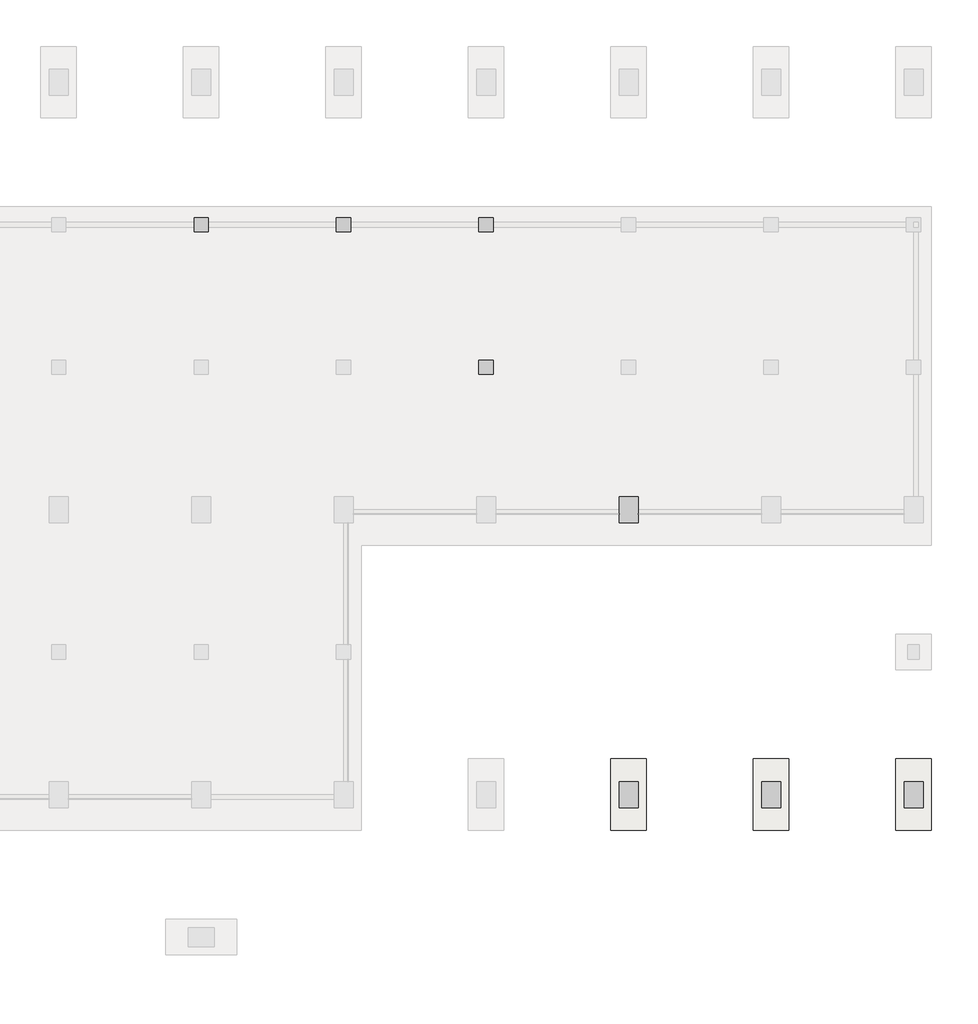
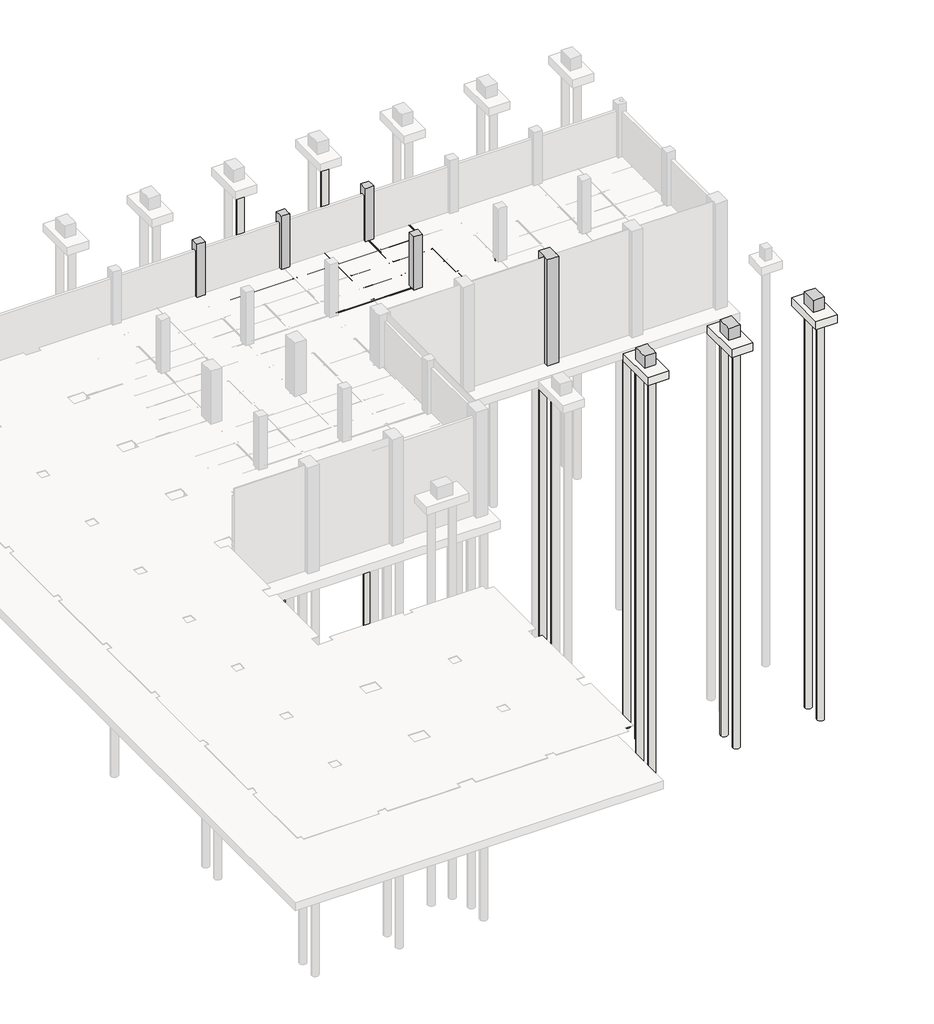
# Not in any storey, part 14 of 16: 21 beams, 17 slabs, 8 columns.
"""IFC4 building model written with IfcOpenShell, lengths in millimetres."""

from ifc_helpers import new_model, si_unit, point, frame, frame_2d, origin, place, context, project, spatial, polyline, circle_curve, trimmed, segment, composite_curve, outline, extrude, faceted_brep, element, save

model = new_model("IFC4")

# Units and contexts
model_context = context("Model", 3, world=origin())
ifc_project = project(units=[si_unit("LENGTHUNIT", "METRE", prefix="MILLI")], contexts=[model_context])

# Site, building
site = spatial("IfcSite", under=ifc_project)
building = spatial("IfcBuilding", under=site)

# Beams
placement = place(None, origin())
element("IfcBeam", 1, ObjectType="Steel Framing_C_KS : H_SB_AR_S02_C-150x75x6.5x10_J1", at=placement, inside=building, context=model_context, shape_type="SweptSolid", body=[
    extrude(outline(composite_curve([segment(polyline([(-7477.2, -3800.0381366), (-7477.2, -3950.0381366), (-7552.2, -3950.0381366)]), True, "CONTINUOUS"), segment(trimmed(circle_curve(frame_2d((-7542.2, -3950.0381366)), 10.0), [point((-7552.2, -3950.0381366))], [point((-7542.2, -3940.0381366))], False, "CARTESIAN"), True, "CONTINUOUS"), segment(polyline([(-7542.2, -3940.0381366), (-7483.7, -3930.7726469), (-7483.7, -3819.3036264), (-7542.2, -3810.0381366)]), True, "CONTINUOUS"), segment(trimmed(circle_curve(frame_2d((-7542.2, -3800.0381366)), 10.0), [point((-7542.2, -3810.0381366))], [point((-7552.2, -3800.0381366))], False, "CARTESIAN"), True, "CONTINUOUS"), segment(polyline([(-7552.2, -3800.0381366), (-7477.2, -3800.0381366)]), True, "CONTINUOUS")], self_intersect=False)), frame((48112.7, 0.0, 0.0), z_axis=(1.0, 0.0, 0.0), x_axis=(0.0, 1.0, 0.0)), (0.0, 0.0, 1.0), 2774.6),
])
element("IfcBeam", 2, ObjectType="Steel Framing_C_KS : H_SB_AR_S02_C-150x75x6.5x10_J1", at=placement, inside=building, context=model_context, shape_type="SweptSolid", body=[
    extrude(outline(composite_curve([segment(polyline([(-7477.2, -3800.0381366), (-7477.2, -3950.0381366), (-7552.2, -3950.0381366)]), True, "CONTINUOUS"), segment(trimmed(circle_curve(frame_2d((-7542.2, -3950.0381366)), 10.0), [point((-7552.2, -3950.0381366))], [point((-7542.2, -3940.0381366))], False, "CARTESIAN"), True, "CONTINUOUS"), segment(polyline([(-7542.2, -3940.0381366), (-7483.7, -3930.7726469), (-7483.7, -3819.3036264), (-7542.2, -3810.0381366)]), True, "CONTINUOUS"), segment(trimmed(circle_curve(frame_2d((-7542.2, -3800.0381366)), 10.0), [point((-7542.2, -3810.0381366))], [point((-7552.2, -3800.0381366))], False, "CARTESIAN"), True, "CONTINUOUS"), segment(polyline([(-7552.2, -3800.0381366), (-7477.2, -3800.0381366)]), True, "CONTINUOUS")], self_intersect=False)), frame((51112.7, 0.0, 0.0), z_axis=(1.0, 0.0, 0.0), x_axis=(0.0, 1.0, 0.0)), (0.0, 0.0, 1.0), 2774.6),
])
element("IfcBeam", 3, ObjectType="Steel Framing_H_KS : H_SB_AR_S02_H-400x200x8x13_BSG1", at=placement, inside=building, context=model_context, shape_type="SweptSolid", body=[
    extrude(outline(composite_curve([segment(polyline([(-11900.0, -4187.0381366), (-11900.0, -4200.0381366), (-12100.0, -4200.0381366), (-12100.0, -4187.0381366), (-12020.0, -4187.0381366)]), True, "CONTINUOUS"), segment(trimmed(circle_curve(frame_2d((-12020.0, -4171.0381366)), 16.0), [point((-12020.0, -4187.0381366))], [point((-12004.0, -4171.0381366))], True, "CARTESIAN"), True, "CONTINUOUS"), segment(polyline([(-12004.0, -4171.0381366), (-12004.0, -3829.0381366)]), True, "CONTINUOUS"), segment(trimmed(circle_curve(frame_2d((-12020.0, -3829.0381366)), 16.0), [point((-12004.0, -3829.0381366))], [point((-12020.0, -3813.0381366))], True, "CARTESIAN"), True, "CONTINUOUS"), segment(polyline([(-12020.0, -3813.0381366), (-12100.0, -3813.0381366), (-12100.0, -3800.0381366), (-11900.0, -3800.0381366), (-11900.0, -3813.0381366), (-11980.0, -3813.0381366)]), True, "CONTINUOUS"), segment(trimmed(circle_curve(frame_2d((-11980.0, -3829.0381366)), 16.0), [point((-11980.0, -3813.0381366))], [point((-11996.0, -3829.0381366))], True, "CARTESIAN"), True, "CONTINUOUS"), segment(polyline([(-11996.0, -3829.0381366), (-11996.0, -4171.0381366)]), True, "CONTINUOUS"), segment(trimmed(circle_curve(frame_2d((-11980.0, -4171.0381366)), 16.0), [point((-11996.0, -4171.0381366))], [point((-11980.0, -4187.0381366))], True, "CARTESIAN"), True, "CONTINUOUS"), segment(polyline([(-11980.0, -4187.0381366), (-11900.0, -4187.0381366)]), True, "CONTINUOUS")], self_intersect=False)), frame((54312.7, 0.0, 0.0), z_axis=(1.0, 0.0, 0.0), x_axis=(0.0, 1.0, 0.0)), (0.0, 0.0, 1.0), 5374.6),
])
element("IfcBeam", 4, ObjectType="Steel Framing_H_KS : H_SB_AR_S02_H-400x200x8x13_BSG2", at=placement, inside=building, context=model_context, shape_type="SweptSolid", body=[
    extrude(outline(composite_curve([segment(polyline([(-4187.0381366, 59900.0), (-4200.0381366, 59900.0), (-4200.0381366, 60100.0), (-4187.0381366, 60100.0), (-4187.0381366, 60020.0)]), True, "CONTINUOUS"), segment(trimmed(circle_curve(frame_2d((-4171.0381366, 60020.0)), 16.0), [point((-4187.0381366, 60020.0))], [point((-4171.0381366, 60004.0))], True, "CARTESIAN"), True, "CONTINUOUS"), segment(polyline([(-4171.0381366, 60004.0), (-3829.0381366, 60004.0)]), True, "CONTINUOUS"), segment(trimmed(circle_curve(frame_2d((-3829.0381366, 60020.0)), 16.0), [point((-3829.0381366, 60004.0))], [point((-3813.0381366, 60020.0))], True, "CARTESIAN"), True, "CONTINUOUS"), segment(polyline([(-3813.0381366, 60020.0), (-3813.0381366, 60100.0), (-3800.0381366, 60100.0), (-3800.0381366, 59900.0), (-3813.0381366, 59900.0), (-3813.0381366, 59980.0)]), True, "CONTINUOUS"), segment(trimmed(circle_curve(frame_2d((-3829.0381366, 59980.0)), 16.0), [point((-3813.0381366, 59980.0))], [point((-3829.0381366, 59996.0))], True, "CARTESIAN"), True, "CONTINUOUS"), segment(polyline([(-3829.0381366, 59996.0), (-4171.0381366, 59996.0)]), True, "CONTINUOUS"), segment(trimmed(circle_curve(frame_2d((-4171.0381366, 59980.0)), 16.0), [point((-4171.0381366, 59996.0))], [point((-4187.0381366, 59980.0))], True, "CARTESIAN"), True, "CONTINUOUS"), segment(polyline([(-4187.0381366, 59980.0), (-4187.0381366, 59900.0)]), True, "CONTINUOUS")], self_intersect=False)), frame((0.0, -11687.3, 0.0), z_axis=(0.0, 1.0, 0.0), x_axis=(0.0, 0.0, 1.0)), (0.0, 0.0, 1.0), 5374.6),
])
element("IfcBeam", 5, ObjectType="Steel Framing_H_KS : H_SB_AR_S02_H-400x200x8x13_BSB1", at=placement, inside=building, context=model_context, shape_type="SweptSolid", body=[
    extrude(outline(composite_curve([segment(polyline([(-4187.0381366, 56900.0), (-4200.0381366, 56900.0), (-4200.0381366, 57100.0), (-4187.0381366, 57100.0), (-4187.0381366, 57020.0)]), True, "CONTINUOUS"), segment(trimmed(circle_curve(frame_2d((-4171.0381366, 57020.0)), 16.0), [point((-4187.0381366, 57020.0))], [point((-4171.0381366, 57004.0))], True, "CARTESIAN"), True, "CONTINUOUS"), segment(polyline([(-4171.0381366, 57004.0), (-3829.0381366, 57004.0)]), True, "CONTINUOUS"), segment(trimmed(circle_curve(frame_2d((-3829.0381366, 57020.0)), 16.0), [point((-3829.0381366, 57004.0))], [point((-3813.0381366, 57020.0))], True, "CARTESIAN"), True, "CONTINUOUS"), segment(polyline([(-3813.0381366, 57020.0), (-3813.0381366, 57100.0), (-3800.0381366, 57100.0), (-3800.0381366, 56900.0), (-3813.0381366, 56900.0), (-3813.0381366, 56980.0)]), True, "CONTINUOUS"), segment(trimmed(circle_curve(frame_2d((-3829.0381366, 56980.0)), 16.0), [point((-3813.0381366, 56980.0))], [point((-3829.0381366, 56996.0))], True, "CARTESIAN"), True, "CONTINUOUS"), segment(polyline([(-3829.0381366, 56996.0), (-4171.0381366, 56996.0)]), True, "CONTINUOUS"), segment(trimmed(circle_curve(frame_2d((-4171.0381366, 56980.0)), 16.0), [point((-4171.0381366, 56996.0))], [point((-4187.0381366, 56980.0))], True, "CARTESIAN"), True, "CONTINUOUS"), segment(polyline([(-4187.0381366, 56980.0), (-4187.0381366, 56900.0)]), True, "CONTINUOUS")], self_intersect=False)), frame((0.0, -11887.3, 0.0), z_axis=(0.0, 1.0, 0.0), x_axis=(0.0, 0.0, 1.0)), (0.0, 0.0, 1.0), 5887.3),
])
element("IfcBeam", 6, ObjectType="Steel Framing_C_KS : H_SB_AR_S02_C-150x75x6.5x10_J1", at=placement, inside=building, context=model_context, shape_type="SweptSolid", body=[
    extrude(outline(composite_curve([segment(polyline([(-7477.2, -3800.0381366), (-7477.2, -3950.0381366), (-7552.2, -3950.0381366)]), True, "CONTINUOUS"), segment(trimmed(circle_curve(frame_2d((-7542.2, -3950.0381366)), 10.0), [point((-7552.2, -3950.0381366))], [point((-7542.2, -3940.0381366))], False, "CARTESIAN"), True, "CONTINUOUS"), segment(polyline([(-7542.2, -3940.0381366), (-7483.7, -3930.7726469), (-7483.7, -3819.3036264), (-7542.2, -3810.0381366)]), True, "CONTINUOUS"), segment(trimmed(circle_curve(frame_2d((-7542.2, -3800.0381366)), 10.0), [point((-7542.2, -3810.0381366))], [point((-7552.2, -3800.0381366))], False, "CARTESIAN"), True, "CONTINUOUS"), segment(polyline([(-7552.2, -3800.0381366), (-7477.2, -3800.0381366)]), True, "CONTINUOUS")], self_intersect=False)), frame((54112.7, 0.0, 0.0), z_axis=(1.0, 0.0, 0.0), x_axis=(0.0, 1.0, 0.0)), (0.0, 0.0, 1.0), 2774.6),
])
element("IfcBeam", 7, ObjectType="Steel Framing_C_KS : H_SB_AR_S02_C-150x75x6.5x10_J1", at=placement, inside=building, context=model_context, shape_type="SweptSolid", body=[
    extrude(outline(composite_curve([segment(polyline([(-8977.2, -3800.0381366), (-8977.2, -3950.0381366), (-9052.2, -3950.0381366)]), True, "CONTINUOUS"), segment(trimmed(circle_curve(frame_2d((-9042.2, -3950.0381366)), 10.0), [point((-9052.2, -3950.0381366))], [point((-9042.2, -3940.0381366))], False, "CARTESIAN"), True, "CONTINUOUS"), segment(polyline([(-9042.2, -3940.0381366), (-8983.7, -3930.7726469), (-8983.7, -3819.3036264), (-9042.2, -3810.0381366)]), True, "CONTINUOUS"), segment(trimmed(circle_curve(frame_2d((-9042.2, -3800.0381366)), 10.0), [point((-9042.2, -3810.0381366))], [point((-9052.2, -3800.0381366))], False, "CARTESIAN"), True, "CONTINUOUS"), segment(polyline([(-9052.2, -3800.0381366), (-8977.2, -3800.0381366)]), True, "CONTINUOUS")], self_intersect=False)), frame((57112.7, 0.0, 0.0), z_axis=(1.0, 0.0, 0.0), x_axis=(0.0, 1.0, 0.0)), (0.0, 0.0, 1.0), 2774.6),
])
element("IfcBeam", 8, ObjectType="Steel Framing_C_KS : H_SB_AR_S02_C-150x75x6.5x10_J1", at=placement, inside=building, context=model_context, shape_type="SweptSolid", body=[
    extrude(outline(composite_curve([segment(polyline([(-10477.2, -3800.0381366), (-10477.2, -3950.0381366), (-10552.2, -3950.0381366)]), True, "CONTINUOUS"), segment(trimmed(circle_curve(frame_2d((-10542.2, -3950.0381366)), 10.0), [point((-10552.2, -3950.0381366))], [point((-10542.2, -3940.0381366))], False, "CARTESIAN"), True, "CONTINUOUS"), segment(polyline([(-10542.2, -3940.0381366), (-10483.7, -3930.7726469), (-10483.7, -3819.3036264), (-10542.2, -3810.0381366)]), True, "CONTINUOUS"), segment(trimmed(circle_curve(frame_2d((-10542.2, -3800.0381366)), 10.0), [point((-10542.2, -3810.0381366))], [point((-10552.2, -3800.0381366))], False, "CARTESIAN"), True, "CONTINUOUS"), segment(polyline([(-10552.2, -3800.0381366), (-10477.2, -3800.0381366)]), True, "CONTINUOUS")], self_intersect=False)), frame((57112.7, 0.0, 0.0), z_axis=(1.0, 0.0, 0.0), x_axis=(0.0, 1.0, 0.0)), (0.0, 0.0, 1.0), 2774.6),
])
element("IfcBeam", 9, ObjectType="Steel Framing_C_KS : H_SB_AR_S02_C-150x75x6.5x10_J1", at=placement, inside=building, context=model_context, shape_type="SweptSolid", body=[
    extrude(outline(composite_curve([segment(polyline([(-7477.2, -3800.0381366), (-7477.2, -3950.0381366), (-7552.2, -3950.0381366)]), True, "CONTINUOUS"), segment(trimmed(circle_curve(frame_2d((-7542.2, -3950.0381366)), 10.0), [point((-7552.2, -3950.0381366))], [point((-7542.2, -3940.0381366))], False, "CARTESIAN"), True, "CONTINUOUS"), segment(polyline([(-7542.2, -3940.0381366), (-7483.7, -3930.7726469), (-7483.7, -3819.3036264), (-7542.2, -3810.0381366)]), True, "CONTINUOUS"), segment(trimmed(circle_curve(frame_2d((-7542.2, -3800.0381366)), 10.0), [point((-7542.2, -3810.0381366))], [point((-7552.2, -3800.0381366))], False, "CARTESIAN"), True, "CONTINUOUS"), segment(polyline([(-7552.2, -3800.0381366), (-7477.2, -3800.0381366)]), True, "CONTINUOUS")], self_intersect=False)), frame((57112.7, 0.0, 0.0), z_axis=(1.0, 0.0, 0.0), x_axis=(0.0, 1.0, 0.0)), (0.0, 0.0, 1.0), 2774.6),
])
element("IfcBeam", 10, ObjectType="Steel Framing_H_KS : H_SB_AR_S02_H-400x200x8x13_BSG1", at=placement, inside=building, context=model_context, shape_type="SweptSolid", body=[
    extrude(outline(composite_curve([segment(polyline([(-11900.0, -4187.0381366), (-11900.0, -4200.0381366), (-12100.0, -4200.0381366), (-12100.0, -4187.0381366), (-12020.0, -4187.0381366)]), True, "CONTINUOUS"), segment(trimmed(circle_curve(frame_2d((-12020.0, -4171.0381366)), 16.0), [point((-12020.0, -4187.0381366))], [point((-12004.0, -4171.0381366))], True, "CARTESIAN"), True, "CONTINUOUS"), segment(polyline([(-12004.0, -4171.0381366), (-12004.0, -3829.0381366)]), True, "CONTINUOUS"), segment(trimmed(circle_curve(frame_2d((-12020.0, -3829.0381366)), 16.0), [point((-12004.0, -3829.0381366))], [point((-12020.0, -3813.0381366))], True, "CARTESIAN"), True, "CONTINUOUS"), segment(polyline([(-12020.0, -3813.0381366), (-12100.0, -3813.0381366), (-12100.0, -3800.0381366), (-11900.0, -3800.0381366), (-11900.0, -3813.0381366), (-11980.0, -3813.0381366)]), True, "CONTINUOUS"), segment(trimmed(circle_curve(frame_2d((-11980.0, -3829.0381366)), 16.0), [point((-11980.0, -3813.0381366))], [point((-11996.0, -3829.0381366))], True, "CARTESIAN"), True, "CONTINUOUS"), segment(polyline([(-11996.0, -3829.0381366), (-11996.0, -4171.0381366)]), True, "CONTINUOUS"), segment(trimmed(circle_curve(frame_2d((-11980.0, -4171.0381366)), 16.0), [point((-11996.0, -4171.0381366))], [point((-11980.0, -4187.0381366))], True, "CARTESIAN"), True, "CONTINUOUS"), segment(polyline([(-11980.0, -4187.0381366), (-11900.0, -4187.0381366)]), True, "CONTINUOUS")], self_intersect=False)), frame((60312.7, 0.0, 0.0), z_axis=(1.0, 0.0, 0.0), x_axis=(0.0, 1.0, 0.0)), (0.0, 0.0, 1.0), 5374.6),
])
element("IfcBeam", 11, ObjectType="Steel Framing_H_KS : H_SB_AR_S02_H-400x200x8x13_BSB1", at=placement, inside=building, context=model_context, shape_type="SweptSolid", body=[
    extrude(outline(composite_curve([segment(polyline([(-4187.0381366, 62900.0), (-4200.0381366, 62900.0), (-4200.0381366, 63100.0), (-4187.0381366, 63100.0), (-4187.0381366, 63020.0)]), True, "CONTINUOUS"), segment(trimmed(circle_curve(frame_2d((-4171.0381366, 63020.0)), 16.0), [point((-4187.0381366, 63020.0))], [point((-4171.0381366, 63004.0))], True, "CARTESIAN"), True, "CONTINUOUS"), segment(polyline([(-4171.0381366, 63004.0), (-3829.0381366, 63004.0)]), True, "CONTINUOUS"), segment(trimmed(circle_curve(frame_2d((-3829.0381366, 63020.0)), 16.0), [point((-3829.0381366, 63004.0))], [point((-3813.0381366, 63020.0))], True, "CARTESIAN"), True, "CONTINUOUS"), segment(polyline([(-3813.0381366, 63020.0), (-3813.0381366, 63100.0), (-3800.0381366, 63100.0), (-3800.0381366, 62900.0), (-3813.0381366, 62900.0), (-3813.0381366, 62980.0)]), True, "CONTINUOUS"), segment(trimmed(circle_curve(frame_2d((-3829.0381366, 62980.0)), 16.0), [point((-3813.0381366, 62980.0))], [point((-3829.0381366, 62996.0))], True, "CARTESIAN"), True, "CONTINUOUS"), segment(polyline([(-3829.0381366, 62996.0), (-4171.0381366, 62996.0)]), True, "CONTINUOUS"), segment(trimmed(circle_curve(frame_2d((-4171.0381366, 62980.0)), 16.0), [point((-4171.0381366, 62996.0))], [point((-4187.0381366, 62980.0))], True, "CARTESIAN"), True, "CONTINUOUS"), segment(polyline([(-4187.0381366, 62980.0), (-4187.0381366, 62900.0)]), True, "CONTINUOUS")], self_intersect=False)), frame((0.0, -11887.3, 0.0), z_axis=(0.0, 1.0, 0.0), x_axis=(0.0, 0.0, 1.0)), (0.0, 0.0, 1.0), 5887.3),
])
element("IfcBeam", 12, ObjectType="Steel Framing_C_KS : H_SB_AR_S02_C-150x75x6.5x10_J1", at=placement, inside=building, context=model_context, shape_type="SweptSolid", body=[
    extrude(outline(composite_curve([segment(polyline([(-8977.2, -3800.0381366), (-8977.2, -3950.0381366), (-9052.2, -3950.0381366)]), True, "CONTINUOUS"), segment(trimmed(circle_curve(frame_2d((-9042.2, -3950.0381366)), 10.0), [point((-9052.2, -3950.0381366))], [point((-9042.2, -3940.0381366))], False, "CARTESIAN"), True, "CONTINUOUS"), segment(polyline([(-9042.2, -3940.0381366), (-8983.7, -3930.7726469), (-8983.7, -3819.3036264), (-9042.2, -3810.0381366)]), True, "CONTINUOUS"), segment(trimmed(circle_curve(frame_2d((-9042.2, -3800.0381366)), 10.0), [point((-9042.2, -3810.0381366))], [point((-9052.2, -3800.0381366))], False, "CARTESIAN"), True, "CONTINUOUS"), segment(polyline([(-9052.2, -3800.0381366), (-8977.2, -3800.0381366)]), True, "CONTINUOUS")], self_intersect=False)), frame((60112.7, 0.0, 0.0), z_axis=(1.0, 0.0, 0.0), x_axis=(0.0, 1.0, 0.0)), (0.0, 0.0, 1.0), 2774.6),
])
element("IfcBeam", 13, ObjectType="Steel Framing_C_KS : H_SB_AR_S02_C-150x75x6.5x10_J1", at=placement, inside=building, context=model_context, shape_type="SweptSolid", body=[
    extrude(outline(composite_curve([segment(polyline([(-10477.2, -3800.0381366), (-10477.2, -3950.0381366), (-10552.2, -3950.0381366)]), True, "CONTINUOUS"), segment(trimmed(circle_curve(frame_2d((-10542.2, -3950.0381366)), 10.0), [point((-10552.2, -3950.0381366))], [point((-10542.2, -3940.0381366))], False, "CARTESIAN"), True, "CONTINUOUS"), segment(polyline([(-10542.2, -3940.0381366), (-10483.7, -3930.7726469), (-10483.7, -3819.3036264), (-10542.2, -3810.0381366)]), True, "CONTINUOUS"), segment(trimmed(circle_curve(frame_2d((-10542.2, -3800.0381366)), 10.0), [point((-10542.2, -3810.0381366))], [point((-10552.2, -3800.0381366))], False, "CARTESIAN"), True, "CONTINUOUS"), segment(polyline([(-10552.2, -3800.0381366), (-10477.2, -3800.0381366)]), True, "CONTINUOUS")], self_intersect=False)), frame((60112.7, 0.0, 0.0), z_axis=(1.0, 0.0, 0.0), x_axis=(0.0, 1.0, 0.0)), (0.0, 0.0, 1.0), 2774.6),
])
element("IfcBeam", 14, ObjectType="Steel Framing_C_KS : H_SB_AR_S02_C-150x75x6.5x10_J1", at=placement, inside=building, context=model_context, shape_type="SweptSolid", body=[
    extrude(outline(composite_curve([segment(polyline([(-7477.2, -3800.0381366), (-7477.2, -3950.0381366), (-7552.2, -3950.0381366)]), True, "CONTINUOUS"), segment(trimmed(circle_curve(frame_2d((-7542.2, -3950.0381366)), 10.0), [point((-7552.2, -3950.0381366))], [point((-7542.2, -3940.0381366))], False, "CARTESIAN"), True, "CONTINUOUS"), segment(polyline([(-7542.2, -3940.0381366), (-7483.7, -3930.7726469), (-7483.7, -3819.3036264), (-7542.2, -3810.0381366)]), True, "CONTINUOUS"), segment(trimmed(circle_curve(frame_2d((-7542.2, -3800.0381366)), 10.0), [point((-7542.2, -3810.0381366))], [point((-7552.2, -3800.0381366))], False, "CARTESIAN"), True, "CONTINUOUS"), segment(polyline([(-7552.2, -3800.0381366), (-7477.2, -3800.0381366)]), True, "CONTINUOUS")], self_intersect=False)), frame((60112.7, 0.0, 0.0), z_axis=(1.0, 0.0, 0.0), x_axis=(0.0, 1.0, 0.0)), (0.0, 0.0, 1.0), 2774.6),
])
element("IfcBeam", 15, ObjectType="Steel Framing_H_KS : H_SB_AR_S02_H-400x200x8x13_BSG2", at=placement, inside=building, context=model_context, shape_type="SweptSolid", body=[
    extrude(outline(composite_curve([segment(polyline([(-4187.0381366, 59900.0), (-4200.0381366, 59900.0), (-4200.0381366, 60100.0), (-4187.0381366, 60100.0), (-4187.0381366, 60020.0)]), True, "CONTINUOUS"), segment(trimmed(circle_curve(frame_2d((-4171.0381366, 60020.0)), 16.0), [point((-4187.0381366, 60020.0))], [point((-4171.0381366, 60004.0))], True, "CARTESIAN"), True, "CONTINUOUS"), segment(polyline([(-4171.0381366, 60004.0), (-3829.0381366, 60004.0)]), True, "CONTINUOUS"), segment(trimmed(circle_curve(frame_2d((-3829.0381366, 60020.0)), 16.0), [point((-3829.0381366, 60004.0))], [point((-3813.0381366, 60020.0))], True, "CARTESIAN"), True, "CONTINUOUS"), segment(polyline([(-3813.0381366, 60020.0), (-3813.0381366, 60100.0), (-3800.0381366, 60100.0), (-3800.0381366, 59900.0), (-3813.0381366, 59900.0), (-3813.0381366, 59980.0)]), True, "CONTINUOUS"), segment(trimmed(circle_curve(frame_2d((-3829.0381366, 59980.0)), 16.0), [point((-3813.0381366, 59980.0))], [point((-3829.0381366, 59996.0))], True, "CARTESIAN"), True, "CONTINUOUS"), segment(polyline([(-3829.0381366, 59996.0), (-4171.0381366, 59996.0)]), True, "CONTINUOUS"), segment(trimmed(circle_curve(frame_2d((-4171.0381366, 59980.0)), 16.0), [point((-4171.0381366, 59996.0))], [point((-4187.0381366, 59980.0))], True, "CARTESIAN"), True, "CONTINUOUS"), segment(polyline([(-4187.0381366, 59980.0), (-4187.0381366, 59900.0)]), True, "CONTINUOUS")], self_intersect=False)), frame((0.0, -17437.3, 0.0), z_axis=(0.0, 1.0, 0.0), x_axis=(0.0, 0.0, 1.0)), (0.0, 0.0, 1.0), 5124.6),
])
element("IfcBeam", 16, ObjectType="Steel Framing_H_KS : H_SB_AR_S02_H-400x200x8x13_BSB1", at=placement, inside=building, context=model_context, shape_type="SweptSolid", body=[
    extrude(outline(composite_curve([segment(polyline([(-4187.0381366, 62900.0), (-4200.0381366, 62900.0), (-4200.0381366, 63100.0), (-4187.0381366, 63100.0), (-4187.0381366, 63020.0)]), True, "CONTINUOUS"), segment(trimmed(circle_curve(frame_2d((-4171.0381366, 63020.0)), 16.0), [point((-4187.0381366, 63020.0))], [point((-4171.0381366, 63004.0))], True, "CARTESIAN"), True, "CONTINUOUS"), segment(polyline([(-4171.0381366, 63004.0), (-3829.0381366, 63004.0)]), True, "CONTINUOUS"), segment(trimmed(circle_curve(frame_2d((-3829.0381366, 63020.0)), 16.0), [point((-3829.0381366, 63004.0))], [point((-3813.0381366, 63020.0))], True, "CARTESIAN"), True, "CONTINUOUS"), segment(polyline([(-3813.0381366, 63020.0), (-3813.0381366, 63100.0), (-3800.0381366, 63100.0), (-3800.0381366, 62900.0), (-3813.0381366, 62900.0), (-3813.0381366, 62980.0)]), True, "CONTINUOUS"), segment(trimmed(circle_curve(frame_2d((-3829.0381366, 62980.0)), 16.0), [point((-3813.0381366, 62980.0))], [point((-3829.0381366, 62996.0))], True, "CARTESIAN"), True, "CONTINUOUS"), segment(polyline([(-3829.0381366, 62996.0), (-4171.0381366, 62996.0)]), True, "CONTINUOUS"), segment(trimmed(circle_curve(frame_2d((-4171.0381366, 62980.0)), 16.0), [point((-4171.0381366, 62996.0))], [point((-4187.0381366, 62980.0))], True, "CARTESIAN"), True, "CONTINUOUS"), segment(polyline([(-4187.0381366, 62980.0), (-4187.0381366, 62900.0)]), True, "CONTINUOUS")], self_intersect=False)), frame((0.0, -18000.0, 0.0), z_axis=(0.0, 1.0, 0.0), x_axis=(0.0, 0.0, 1.0)), (0.0, 0.0, 1.0), 5887.3),
])
element("IfcBeam", 17, ObjectType="Steel Framing_C_KS : H_SB_AR_S02_C-150x75x6.5x10_J1", at=placement, inside=building, context=model_context, shape_type="SweptSolid", body=[
    extrude(outline(composite_curve([segment(polyline([(-14977.2, -3800.0381366), (-14977.2, -3950.0381366), (-15052.2, -3950.0381366)]), True, "CONTINUOUS"), segment(trimmed(circle_curve(frame_2d((-15042.2, -3950.0381366)), 10.0), [point((-15052.2, -3950.0381366))], [point((-15042.2, -3940.0381366))], False, "CARTESIAN"), True, "CONTINUOUS"), segment(polyline([(-15042.2, -3940.0381366), (-14983.7, -3930.7726469), (-14983.7, -3819.3036264), (-15042.2, -3810.0381366)]), True, "CONTINUOUS"), segment(trimmed(circle_curve(frame_2d((-15042.2, -3800.0381366)), 10.0), [point((-15042.2, -3810.0381366))], [point((-15052.2, -3800.0381366))], False, "CARTESIAN"), True, "CONTINUOUS"), segment(polyline([(-15052.2, -3800.0381366), (-14977.2, -3800.0381366)]), True, "CONTINUOUS")], self_intersect=False)), frame((60112.7, 0.0, 0.0), z_axis=(1.0, 0.0, 0.0), x_axis=(0.0, 1.0, 0.0)), (0.0, 0.0, 1.0), 2774.6),
])
element("IfcBeam", 18, ObjectType="Steel Framing_C_KS : H_SB_AR_S02_C-150x75x6.5x10_J1", at=placement, inside=building, context=model_context, shape_type="SweptSolid", body=[
    extrude(outline(composite_curve([segment(polyline([(-13477.2, -3800.0381366), (-13477.2, -3950.0381366), (-13552.2, -3950.0381366)]), True, "CONTINUOUS"), segment(trimmed(circle_curve(frame_2d((-13542.2, -3950.0381366)), 10.0), [point((-13552.2, -3950.0381366))], [point((-13542.2, -3940.0381366))], False, "CARTESIAN"), True, "CONTINUOUS"), segment(polyline([(-13542.2, -3940.0381366), (-13483.7, -3930.7726469), (-13483.7, -3819.3036264), (-13542.2, -3810.0381366)]), True, "CONTINUOUS"), segment(trimmed(circle_curve(frame_2d((-13542.2, -3800.0381366)), 10.0), [point((-13542.2, -3810.0381366))], [point((-13552.2, -3800.0381366))], False, "CARTESIAN"), True, "CONTINUOUS"), segment(polyline([(-13552.2, -3800.0381366), (-13477.2, -3800.0381366)]), True, "CONTINUOUS")], self_intersect=False)), frame((60112.7, 0.0, 0.0), z_axis=(1.0, 0.0, 0.0), x_axis=(0.0, 1.0, 0.0)), (0.0, 0.0, 1.0), 2774.6),
])
element("IfcBeam", 19, ObjectType="Steel Framing_C_KS : H_SB_AR_S02_C-150x75x6.5x10_J1", at=placement, inside=building, context=model_context, shape_type="SweptSolid", body=[
    extrude(outline(composite_curve([segment(polyline([(-16477.2, -3800.0381366), (-16477.2, -3950.0381366), (-16552.2, -3950.0381366)]), True, "CONTINUOUS"), segment(trimmed(circle_curve(frame_2d((-16542.2, -3950.0381366)), 10.0), [point((-16552.2, -3950.0381366))], [point((-16542.2, -3940.0381366))], False, "CARTESIAN"), True, "CONTINUOUS"), segment(polyline([(-16542.2, -3940.0381366), (-16483.7, -3930.7726469), (-16483.7, -3819.3036264), (-16542.2, -3810.0381366)]), True, "CONTINUOUS"), segment(trimmed(circle_curve(frame_2d((-16542.2, -3800.0381366)), 10.0), [point((-16542.2, -3810.0381366))], [point((-16552.2, -3800.0381366))], False, "CARTESIAN"), True, "CONTINUOUS"), segment(polyline([(-16552.2, -3800.0381366), (-16477.2, -3800.0381366)]), True, "CONTINUOUS")], self_intersect=False)), frame((63112.7, 0.0, 0.0), z_axis=(1.0, 0.0, 0.0), x_axis=(0.0, 1.0, 0.0)), (0.0, 0.0, 1.0), 2774.6),
])
element("IfcBeam", 20, ObjectType="Steel Framing_C_KS : H_SB_AR_S02_C-150x75x6.5x10_J1", at=placement, inside=building, context=model_context, shape_type="SweptSolid", body=[
    extrude(outline(composite_curve([segment(polyline([(-16477.2, -3800.0381366), (-16477.2, -3950.0381366), (-16552.2, -3950.0381366)]), True, "CONTINUOUS"), segment(trimmed(circle_curve(frame_2d((-16542.2, -3950.0381366)), 10.0), [point((-16552.2, -3950.0381366))], [point((-16542.2, -3940.0381366))], False, "CARTESIAN"), True, "CONTINUOUS"), segment(polyline([(-16542.2, -3940.0381366), (-16483.7, -3930.7726469), (-16483.7, -3819.3036264), (-16542.2, -3810.0381366)]), True, "CONTINUOUS"), segment(trimmed(circle_curve(frame_2d((-16542.2, -3800.0381366)), 10.0), [point((-16542.2, -3810.0381366))], [point((-16552.2, -3800.0381366))], False, "CARTESIAN"), True, "CONTINUOUS"), segment(polyline([(-16552.2, -3800.0381366), (-16477.2, -3800.0381366)]), True, "CONTINUOUS")], self_intersect=False)), frame((66112.7, 0.0, 0.0), z_axis=(1.0, 0.0, 0.0), x_axis=(0.0, 1.0, 0.0)), (0.0, 0.0, 1.0), 2774.6),
])
element("IfcBeam", 21, ObjectType="Steel Framing_C_KS : H_SB_AR_S02_C-150x75x6.5x10_J1", at=placement, inside=building, context=model_context, shape_type="SweptSolid", body=[
    extrude(outline(composite_curve([segment(polyline([(-16477.2, -3800.0381366), (-16477.2, -3950.0381366), (-16552.2, -3950.0381366)]), True, "CONTINUOUS"), segment(trimmed(circle_curve(frame_2d((-16542.2, -3950.0381366)), 10.0), [point((-16552.2, -3950.0381366))], [point((-16542.2, -3940.0381366))], False, "CARTESIAN"), True, "CONTINUOUS"), segment(polyline([(-16542.2, -3940.0381366), (-16483.7, -3930.7726469), (-16483.7, -3819.3036264), (-16542.2, -3810.0381366)]), True, "CONTINUOUS"), segment(trimmed(circle_curve(frame_2d((-16542.2, -3800.0381366)), 10.0), [point((-16542.2, -3810.0381366))], [point((-16552.2, -3800.0381366))], False, "CARTESIAN"), True, "CONTINUOUS"), segment(polyline([(-16552.2, -3800.0381366), (-16477.2, -3800.0381366)]), True, "CONTINUOUS")], self_intersect=False)), frame((69112.7, 0.0, 0.0), z_axis=(1.0, 0.0, 0.0), x_axis=(0.0, 1.0, 0.0)), (0.0, 0.0, 1.0), 2774.6),
])

# Columns
element("IfcColumn", 22, ObjectType="RC_Column_Rectangular : H_SC_AR_S15_UG PED_Bit_800x1100_PD1", at=placement, inside=building, context=model_context, shape_type="Brep", body=[
    faceted_brep([(66400.0, -17450.0, -7800.0381366), (66400.0, -18000.0, -7800.0381366), (66400.0, -18200.0, -7800.0381366), (66400.0, -18550.0, -7800.0381366), (65600.0, -18550.0, -7800.0381366), (65600.0, -18200.0, -7800.0381366), (65600.0, -18000.0, -7800.0381366), (65600.0, -17450.0, -7800.0381366), (66400.0, -17450.0, 199.9618634), (66400.0, -17825.0, 199.9618634), (66400.0, -18000.0, 199.9618634), (66400.0, -18175.0, 199.9618634), (66400.0, -18200.0, 199.9618634), (66400.0, -18550.0, 199.9618634), (66400.0, -18550.0, -0.0381366), (66400.0, -17450.0, -3832.0381366), (66400.0, -17450.0, -3800.0381366), (66400.0, -17450.0, -0.0381366), (65600.0, -18550.0, 199.9618634), (65600.0, -18550.0, -0.0381366), (65600.0, -18200.0, 199.9618634), (65600.0, -18175.0, 199.9618634), (65600.0, -18000.0, 199.9618634), (65600.0, -17825.0, 199.9618634), (65600.0, -17450.0, 199.9618634), (65600.0, -17450.0, -0.0381366), (65600.0, -17450.0, -3800.0381366), (65600.0, -17450.0, -3832.0381366), (65825.0, -17450.0, 199.9618634), (66175.0, -17450.0, 199.9618634)], [[[0, 1, 2, 3, 4, 5, 6, 7]], [[8, 9, 10, 11, 12, 13, 14, 3, 2, 1, 0, 15, 16, 17]], [[13, 18, 19, 4, 3, 14]], [[18, 20, 21, 22, 23, 24, 25, 26, 27, 7, 6, 5, 4, 19]], [[24, 28, 29, 8, 17, 16, 15, 0, 7, 27, 26, 25]], [[8, 29, 28, 24, 23, 22, 21, 20, 18, 13, 12, 11, 10, 9]]]),
])
element("IfcColumn", 23, ObjectType="RC_Column_Rectangular : H_SC_AR_S15_UG PED_Bit_800x1100_PD1", at=placement, inside=building, context=model_context, shape_type="Brep", body=[
    faceted_brep([(66400.0, -29450.0, -700.0381366), (66400.0, -30550.0, -700.0381366), (65600.0, -30550.0, -700.0381366), (65600.0, -29450.0, -700.0381366), (66400.0, -29450.0, 199.9618634), (66400.0, -29800.0, 199.9618634), (66400.0, -30200.0, 199.9618634), (66400.0, -30550.0, 199.9618634), (66400.0, -29450.0, -0.0381366), (65600.0, -30550.0, 199.9618634), (65600.0, -30200.0, 199.9618634), (65600.0, -29800.0, 199.9618634), (65600.0, -29450.0, 199.9618634), (65600.0, -29450.0, -0.0381366)], [[[0, 1, 2, 3]], [[4, 5, 6, 7, 1, 0, 8]], [[7, 9, 2, 1]], [[9, 10, 11, 12, 13, 3, 2]], [[12, 4, 8, 0, 3, 13]], [[4, 12, 11, 10, 9, 7, 6, 5]]]),
])
element("IfcColumn", 24, ObjectType="RC_Column_Rectangular : H_SC_AR_S15_UG PED_Bit_800x1100_PD1", at=placement, inside=building, context=model_context, shape_type="Brep", body=[
    faceted_brep([(72400.0, -29450.0, -700.0381366), (72400.0, -30550.0, -700.0381366), (71600.0, -30550.0, -700.0381366), (71600.0, -29450.0, -700.0381366), (72400.0, -29450.0, 199.9618634), (72400.0, -29800.0, 199.9618634), (72400.0, -30200.0, 199.9618634), (72400.0, -30550.0, 199.9618634), (72400.0, -29450.0, -0.0381366), (71600.0, -30550.0, 199.9618634), (71600.0, -30200.0, 199.9618634), (71600.0, -29800.0, 199.9618634), (71600.0, -29450.0, 199.9618634), (71600.0, -29450.0, -0.0381366)], [[[0, 1, 2, 3]], [[4, 5, 6, 7, 1, 0, 8]], [[7, 9, 2, 1]], [[9, 10, 11, 12, 13, 3, 2]], [[12, 4, 8, 0, 3, 13]], [[4, 12, 11, 10, 9, 7, 6, 5]]]),
])
element("IfcColumn", 25, ObjectType="RC_Column_Rectangular : H_SC_AR_S15_UG PED_Bit_800x1100_PD1", at=placement, inside=building, context=model_context, shape_type="Brep", body=[
    faceted_brep([(78400.0, -29450.0, -700.0381366), (78400.0, -30550.0, -700.0381366), (77600.0, -30550.0, -700.0381366), (77600.0, -29450.0, -700.0381366), (78400.0, -29450.0, 199.9618634), (78400.0, -30550.0, 199.9618634), (77600.0, -30550.0, 199.9618634), (77600.0, -29800.0, 199.9618634), (77600.0, -29450.0, 199.9618634), (77600.0, -29450.0, -0.0381366), (77800.0, -29450.0, 199.9618634)], [[[0, 1, 2, 3]], [[4, 5, 1, 0]], [[5, 6, 2, 1]], [[6, 7, 8, 9, 3, 2]], [[8, 10, 4, 0, 3, 9]], [[4, 10, 8, 7, 6, 5]]]),
])
element("IfcColumn", 26, ObjectType="RC_Column_Rectangular : H_SC_AR_S15_UG PED_Bit_600x600_BC1", at=placement, inside=building, context=model_context, shape_type="Brep", body=[
    faceted_brep([(48300.0, -5700.0, -7800.0381366), (48300.0, -6300.0, -7800.0381366), (47700.0, -6300.0, -7800.0381366), (47700.0, -5700.0, -7800.0381366), (48300.0, -5700.0, 199.9618634), (48300.0, -6100.0, 199.9618634), (48300.0, -6300.0, 199.9618634), (48300.0, -6300.0, -0.0381366), (48300.0, -6300.0, -3800.0381366), (48300.0, -6300.0, -3832.0381366), (48300.0, -5700.0, -0.0381366), (48175.0, -6300.0, 199.9618634), (47825.0, -6300.0, 199.9618634), (47700.0, -6300.0, 199.9618634), (47700.0, -6300.0, -0.0381366), (47700.0, -6300.0, -3800.0381366), (47700.0, -6300.0, -3832.0381366), (47700.0, -6100.0, 199.9618634), (47700.0, -5700.0, 199.9618634), (47700.0, -5700.0, -0.0381366)], [[[0, 1, 2, 3]], [[4, 5, 6, 7, 8, 9, 1, 0, 10]], [[6, 11, 12, 13, 14, 15, 16, 2, 1, 9, 8, 7]], [[13, 17, 18, 19, 3, 2, 16, 15, 14]], [[18, 4, 10, 0, 3, 19]], [[4, 18, 17, 13, 12, 11, 6, 5]]]),
])
element("IfcColumn", 27, ObjectType="RC_Column_Rectangular : H_SC_AR_S15_UG PED_Bit_600x600_BC1", at=placement, inside=building, context=model_context, shape_type="Brep", body=[
    faceted_brep([(54300.0, -5700.0, -7800.0381366), (54300.0, -6300.0, -7800.0381366), (53700.0, -6300.0, -7800.0381366), (53700.0, -5700.0, -7800.0381366), (54300.0, -5700.0, 199.9618634), (54300.0, -6100.0, 199.9618634), (54300.0, -6300.0, 199.9618634), (54300.0, -6300.0, -0.0381366), (54300.0, -6300.0, -3800.0381366), (54300.0, -6300.0, -3832.0381366), (54300.0, -5700.0, -0.0381366), (54175.0, -6300.0, 199.9618634), (53825.0, -6300.0, 199.9618634), (53700.0, -6300.0, 199.9618634), (53700.0, -6300.0, -0.0381366), (53700.0, -6300.0, -3800.0381366), (53700.0, -6300.0, -3832.0381366), (53700.0, -6100.0, 199.9618634), (53700.0, -5700.0, 199.9618634), (53700.0, -5700.0, -0.0381366)], [[[0, 1, 2, 3]], [[4, 5, 6, 7, 8, 9, 1, 0, 10]], [[6, 11, 12, 13, 14, 15, 16, 2, 1, 9, 8, 7]], [[13, 17, 18, 19, 3, 2, 16, 15, 14]], [[18, 4, 10, 0, 3, 19]], [[4, 18, 17, 13, 12, 11, 6, 5]]]),
])
element("IfcColumn", 28, ObjectType="RC_Column_Rectangular : H_SC_AR_S15_UG PED_Bit_600x600_BC1", at=placement, inside=building, context=model_context, shape_type="Brep", body=[
    faceted_brep([(60300.0, -5700.0, -7800.0381366), (60300.0, -6300.0, -7800.0381366), (59700.0, -6300.0, -7800.0381366), (59700.0, -5700.0, -7800.0381366), (60300.0, -5700.0, 199.9618634), (60300.0, -6100.0, 199.9618634), (60300.0, -6300.0, 199.9618634), (60300.0, -6300.0, -0.0381366), (60300.0, -6300.0, -3800.0381366), (60300.0, -6300.0, -3832.0381366), (60300.0, -5700.0, -0.0381366), (60175.0, -6300.0, 199.9618634), (59825.0, -6300.0, 199.9618634), (59700.0, -6300.0, 199.9618634), (59700.0, -6300.0, -0.0381366), (59700.0, -6300.0, -3800.0381366), (59700.0, -6300.0, -3832.0381366), (59700.0, -6100.0, 199.9618634), (59700.0, -5700.0, 199.9618634), (59700.0, -5700.0, -0.0381366)], [[[0, 1, 2, 3]], [[4, 5, 6, 7, 8, 9, 1, 0, 10]], [[6, 11, 12, 13, 14, 15, 16, 2, 1, 9, 8, 7]], [[13, 17, 18, 19, 3, 2, 16, 15, 14]], [[18, 4, 10, 0, 3, 19]], [[4, 18, 17, 13, 12, 11, 6, 5]]]),
])
element("IfcColumn", 29, ObjectType="RC_Column_Rectangular : H_SC_AR_S15_UG PED_Bit_600x600_BC1", at=placement, inside=building, context=model_context, shape_type="Brep", body=[
    faceted_brep([(60300.0, -11700.0, -7200.0381366), (60300.0, -12300.0, -7200.0381366), (59700.0, -12300.0, -7200.0381366), (59700.0, -11700.0, -7200.0381366), (60300.0, -11700.0, 199.9618634), (60300.0, -11825.0, 199.9618634), (60300.0, -12175.0, 199.9618634), (60300.0, -12300.0, 199.9618634), (60300.0, -12300.0, -3800.0381366), (60300.0, -12300.0, -3832.0381366), (60300.0, -11700.0, -3832.0381366), (60300.0, -11700.0, -3800.0381366), (60300.0, -11700.0, -0.0381366), (60175.0, -12300.0, 199.9618634), (59825.0, -12300.0, 199.9618634), (59700.0, -12300.0, 199.9618634), (59700.0, -12300.0, -3800.0381366), (59700.0, -12300.0, -3832.0381366), (59700.0, -12175.0, 199.9618634), (59700.0, -11825.0, 199.9618634), (59700.0, -11700.0, 199.9618634), (59700.0, -11700.0, -0.0381366), (59700.0, -11700.0, -3800.0381366), (59700.0, -11700.0, -3832.0381366), (59825.0, -11700.0, 199.9618634), (60175.0, -11700.0, 199.9618634)], [[[0, 1, 2, 3]], [[4, 5, 6, 7, 8, 9, 1, 0, 10, 11, 12]], [[7, 13, 14, 15, 16, 17, 2, 1, 9, 8]], [[15, 18, 19, 20, 21, 22, 23, 3, 2, 17, 16]], [[20, 24, 25, 4, 12, 11, 10, 0, 3, 23, 22, 21]], [[4, 25, 24, 20, 19, 18, 15, 14, 13, 7, 6, 5]]]),
])

# Slabs
element("IfcSlab", 30, ObjectType="Foundation Rectangular (Non-Pile) : H_SF_AR_S18_Shallow Fdn_Bitumen_1500x3000xT600_F1", at=placement, inside=building, context=model_context, shape_type="SweptSolid", body=[
    extrude(outline(polyline([(66750.0, -28500.0), (66750.0, -31500.0), (65250.0, -31500.0), (65250.0, -28500.0), (66750.0, -28500.0)])), frame((0.0, 0.0, -1300.0381366), z_axis=(0.0, 0.0, 1.0), x_axis=(1.0, 0.0, 0.0)), (0.0, 0.0, 1.0), 600.0),
])
element("IfcSlab", 31, ObjectType="Foundation Rectangular (Non-Pile) : H_SF_AR_S18_Shallow Fdn_Bitumen_1500x3000xT600_F1", at=placement, inside=building, context=model_context, shape_type="SweptSolid", body=[
    extrude(outline(polyline([(72750.0, -28500.0), (72750.0, -31500.0), (71250.0, -31500.0), (71250.0, -28500.0), (72750.0, -28500.0)])), frame((0.0, 0.0, -1300.0381366), z_axis=(0.0, 0.0, 1.0), x_axis=(1.0, 0.0, 0.0)), (0.0, 0.0, 1.0), 600.0),
])
element("IfcSlab", 32, ObjectType="Foundation Rectangular (Non-Pile) : H_SF_AR_S18_Shallow Fdn_Bitumen_1500x3000xT600_F1", at=placement, inside=building, context=model_context, shape_type="SweptSolid", body=[
    extrude(outline(polyline([(78750.0, -28500.0), (78750.0, -31500.0), (77250.0, -31500.0), (77250.0, -28500.0), (78750.0, -28500.0)])), frame((0.0, 0.0, -1300.0381366), z_axis=(0.0, 0.0, 1.0), x_axis=(1.0, 0.0, 0.0)), (0.0, 0.0, 1.0), 600.0),
])
element("IfcSlab", 33, ObjectType="PILE : H_SF_AR_S19_PHC Pile_Pre-boring_D500_L30", at=placement, inside=building, context=model_context, shape_type="SweptSolid", body=[
    extrude(outline(composite_curve([segment(trimmed(circle_curve(frame_2d((54000.0, -750.0)), 250.0), [point((53750.0, -750.0))], [point((54250.0, -750.0))], False, "CARTESIAN"), True, "CONTINUOUS"), segment(trimmed(circle_curve(frame_2d((54000.0, -750.0)), 250.0), [point((54250.0, -750.0))], [point((53750.0, -750.0))], False, "CARTESIAN"), True, "CONTINUOUS")], self_intersect=False)), frame((0.0, 0.0, -31300.0381366), z_axis=(0.0, 0.0, 1.0), x_axis=(1.0, 0.0, 0.0)), (0.0, 0.0, 1.0), 30000.0),
])
element("IfcSlab", 34, ObjectType="PILE : H_SF_AR_S19_PHC Pile_Pre-boring_D500_L30", at=placement, inside=building, context=model_context, shape_type="SweptSolid", body=[
    extrude(outline(composite_curve([segment(trimmed(circle_curve(frame_2d((60000.0, -750.0)), 250.0), [point((59750.0, -750.0))], [point((60250.0, -750.0))], False, "CARTESIAN"), True, "CONTINUOUS"), segment(trimmed(circle_curve(frame_2d((60000.0, -750.0)), 250.0), [point((60250.0, -750.0))], [point((59750.0, -750.0))], False, "CARTESIAN"), True, "CONTINUOUS")], self_intersect=False)), frame((0.0, 0.0, -31300.0381366), z_axis=(0.0, 0.0, 1.0), x_axis=(1.0, 0.0, 0.0)), (0.0, 0.0, 1.0), 30000.0),
])
element("IfcSlab", 35, ObjectType="PILE : H_SF_AR_S19_PHC Pile_Pre-boring_D500_L30", at=placement, inside=building, context=model_context, shape_type="SweptSolid", body=[
    extrude(outline(composite_curve([segment(trimmed(circle_curve(frame_2d((78000.0, -29250.0)), 250.0), [point((77750.0, -29250.0))], [point((78250.0, -29250.0))], False, "CARTESIAN"), True, "CONTINUOUS"), segment(trimmed(circle_curve(frame_2d((78000.0, -29250.0)), 250.0), [point((78250.0, -29250.0))], [point((77750.0, -29250.0))], False, "CARTESIAN"), True, "CONTINUOUS")], self_intersect=False)), frame((0.0, 0.0, -31300.0381366), z_axis=(0.0, 0.0, 1.0), x_axis=(1.0, 0.0, 0.0)), (0.0, 0.0, 1.0), 30000.0),
])
element("IfcSlab", 36, ObjectType="PILE : H_SF_AR_S19_PHC Pile_Pre-boring_D500_L30", at=placement, inside=building, context=model_context, shape_type="SweptSolid", body=[
    extrude(outline(composite_curve([segment(trimmed(circle_curve(frame_2d((78000.0, -30750.0)), 250.0), [point((77750.0, -30750.0))], [point((78250.0, -30750.0))], False, "CARTESIAN"), True, "CONTINUOUS"), segment(trimmed(circle_curve(frame_2d((78000.0, -30750.0)), 250.0), [point((78250.0, -30750.0))], [point((77750.0, -30750.0))], False, "CARTESIAN"), True, "CONTINUOUS")], self_intersect=False)), frame((0.0, 0.0, -31300.0381366), z_axis=(0.0, 0.0, 1.0), x_axis=(1.0, 0.0, 0.0)), (0.0, 0.0, 1.0), 30000.0),
])
element("IfcSlab", 37, ObjectType="PILE : H_SF_AR_S19_PHC Pile_Pre-boring_D500_L30", at=placement, inside=building, context=model_context, shape_type="SweptSolid", body=[
    extrude(outline(composite_curve([segment(trimmed(circle_curve(frame_2d((72000.0, -29250.0)), 250.0), [point((71750.0, -29250.0))], [point((72250.0, -29250.0))], False, "CARTESIAN"), True, "CONTINUOUS"), segment(trimmed(circle_curve(frame_2d((72000.0, -29250.0)), 250.0), [point((72250.0, -29250.0))], [point((71750.0, -29250.0))], False, "CARTESIAN"), True, "CONTINUOUS")], self_intersect=False)), frame((0.0, 0.0, -31300.0381366), z_axis=(0.0, 0.0, 1.0), x_axis=(1.0, 0.0, 0.0)), (0.0, 0.0, 1.0), 30000.0),
])
element("IfcSlab", 38, ObjectType="PILE : H_SF_AR_S19_PHC Pile_Pre-boring_D500_L30", at=placement, inside=building, context=model_context, shape_type="SweptSolid", body=[
    extrude(outline(composite_curve([segment(trimmed(circle_curve(frame_2d((72000.0, -30750.0)), 250.0), [point((71750.0, -30750.0))], [point((72250.0, -30750.0))], False, "CARTESIAN"), True, "CONTINUOUS"), segment(trimmed(circle_curve(frame_2d((72000.0, -30750.0)), 250.0), [point((72250.0, -30750.0))], [point((71750.0, -30750.0))], False, "CARTESIAN"), True, "CONTINUOUS")], self_intersect=False)), frame((0.0, 0.0, -31300.0381366), z_axis=(0.0, 0.0, 1.0), x_axis=(1.0, 0.0, 0.0)), (0.0, 0.0, 1.0), 30000.0),
])
element("IfcSlab", 39, ObjectType="PILE : H_SF_AR_S19_PHC Pile_Pre-boring_D500_L30", at=placement, inside=building, context=model_context, shape_type="SweptSolid", body=[
    extrude(outline(composite_curve([segment(trimmed(circle_curve(frame_2d((66000.0, -29250.0)), 250.0), [point((65750.0, -29250.0))], [point((66250.0, -29250.0))], False, "CARTESIAN"), True, "CONTINUOUS"), segment(trimmed(circle_curve(frame_2d((66000.0, -29250.0)), 250.0), [point((66250.0, -29250.0))], [point((65750.0, -29250.0))], False, "CARTESIAN"), True, "CONTINUOUS")], self_intersect=False)), frame((0.0, 0.0, -31300.0381366), z_axis=(0.0, 0.0, 1.0), x_axis=(1.0, 0.0, 0.0)), (0.0, 0.0, 1.0), 30000.0),
])
element("IfcSlab", 40, ObjectType="PILE : H_SF_AR_S19_PHC Pile_Pre-boring_D500_L30", at=placement, inside=building, context=model_context, shape_type="SweptSolid", body=[
    extrude(outline(composite_curve([segment(trimmed(circle_curve(frame_2d((66000.0, -30750.0)), 250.0), [point((65750.0, -30750.0))], [point((66250.0, -30750.0))], False, "CARTESIAN"), True, "CONTINUOUS"), segment(trimmed(circle_curve(frame_2d((66000.0, -30750.0)), 250.0), [point((66250.0, -30750.0))], [point((65750.0, -30750.0))], False, "CARTESIAN"), True, "CONTINUOUS")], self_intersect=False)), frame((0.0, 0.0, -31300.0381366), z_axis=(0.0, 0.0, 1.0), x_axis=(1.0, 0.0, 0.0)), (0.0, 0.0, 1.0), 30000.0),
])
element("IfcSlab", 41, ObjectType="PILE : H_SF_AR_S19_PHC Pile_Pre-boring_D500_L30", at=placement, inside=building, context=model_context, shape_type="SweptSolid", body=[
    extrude(outline(composite_curve([segment(trimmed(circle_curve(frame_2d((54000.0, -6000.0)), 250.0), [point((53750.0, -6000.0))], [point((54250.0, -6000.0))], False, "CARTESIAN"), True, "CONTINUOUS"), segment(trimmed(circle_curve(frame_2d((54000.0, -6000.0)), 250.0), [point((54250.0, -6000.0))], [point((53750.0, -6000.0))], False, "CARTESIAN"), True, "CONTINUOUS")], self_intersect=False)), frame((0.0, 0.0, -37950.0381366), z_axis=(0.0, 0.0, 1.0), x_axis=(1.0, 0.0, 0.0)), (0.0, 0.0, 1.0), 29550.0),
])
element("IfcSlab", 42, ObjectType="PILE : H_SF_AR_S19_PHC Pile_Pre-boring_D500_L30", at=placement, inside=building, context=model_context, shape_type="SweptSolid", body=[
    extrude(outline(composite_curve([segment(trimmed(circle_curve(frame_2d((60000.0, -6000.0)), 250.0), [point((59750.0, -6000.0))], [point((60250.0, -6000.0))], False, "CARTESIAN"), True, "CONTINUOUS"), segment(trimmed(circle_curve(frame_2d((60000.0, -6000.0)), 250.0), [point((60250.0, -6000.0))], [point((59750.0, -6000.0))], False, "CARTESIAN"), True, "CONTINUOUS")], self_intersect=False)), frame((0.0, 0.0, -37950.0381366), z_axis=(0.0, 0.0, 1.0), x_axis=(1.0, 0.0, 0.0)), (0.0, 0.0, 1.0), 29550.0),
])
element("IfcSlab", 43, ObjectType="PILE : H_SF_AR_S19_PHC Pile_Pre-boring_D500_L30", at=placement, inside=building, context=model_context, shape_type="SweptSolid", body=[
    extrude(outline(composite_curve([segment(trimmed(circle_curve(frame_2d((66000.0, -17250.0)), 250.0), [point((65750.0, -17250.0))], [point((66250.0, -17250.0))], False, "CARTESIAN"), True, "CONTINUOUS"), segment(trimmed(circle_curve(frame_2d((66000.0, -17250.0)), 250.0), [point((66250.0, -17250.0))], [point((65750.0, -17250.0))], False, "CARTESIAN"), True, "CONTINUOUS")], self_intersect=False)), frame((0.0, 0.0, -37950.0381366), z_axis=(0.0, 0.0, 1.0), x_axis=(1.0, 0.0, 0.0)), (0.0, 0.0, 1.0), 29550.0),
])
element("IfcSlab", 44, ObjectType="PILE : H_SF_AR_S19_PHC Pile_Pre-boring_D500_L30", at=placement, inside=building, context=model_context, shape_type="SweptSolid", body=[
    extrude(outline(composite_curve([segment(trimmed(circle_curve(frame_2d((66000.0, -18750.0)), 250.0), [point((65750.0, -18750.0))], [point((66250.0, -18750.0))], False, "CARTESIAN"), True, "CONTINUOUS"), segment(trimmed(circle_curve(frame_2d((66000.0, -18750.0)), 250.0), [point((66250.0, -18750.0))], [point((65750.0, -18750.0))], False, "CARTESIAN"), True, "CONTINUOUS")], self_intersect=False)), frame((0.0, 0.0, -37950.0381366), z_axis=(0.0, 0.0, 1.0), x_axis=(1.0, 0.0, 0.0)), (0.0, 0.0, 1.0), 29550.0),
])
element("IfcSlab", 45, ObjectType="PILE : H_SF_AR_S19_PHC Pile_Pre-boring_D500_L30", at=placement, inside=building, context=model_context, shape_type="SweptSolid", body=[
    extrude(outline(composite_curve([segment(trimmed(circle_curve(frame_2d((72000.0, -17250.0)), 250.0), [point((71750.0, -17250.0))], [point((72250.0, -17250.0))], False, "CARTESIAN"), True, "CONTINUOUS"), segment(trimmed(circle_curve(frame_2d((72000.0, -17250.0)), 250.0), [point((72250.0, -17250.0))], [point((71750.0, -17250.0))], False, "CARTESIAN"), True, "CONTINUOUS")], self_intersect=False)), frame((0.0, 0.0, -37950.0381366), z_axis=(0.0, 0.0, 1.0), x_axis=(1.0, 0.0, 0.0)), (0.0, 0.0, 1.0), 29550.0),
])
element("IfcSlab", 46, ObjectType="PILE : H_SF_AR_S19_PHC Pile_Pre-boring_D500_L30", at=placement, inside=building, context=model_context, shape_type="SweptSolid", body=[
    extrude(outline(composite_curve([segment(trimmed(circle_curve(frame_2d((72000.0, -18750.0)), 250.0), [point((71750.0, -18750.0))], [point((72250.0, -18750.0))], False, "CARTESIAN"), True, "CONTINUOUS"), segment(trimmed(circle_curve(frame_2d((72000.0, -18750.0)), 250.0), [point((72250.0, -18750.0))], [point((71750.0, -18750.0))], False, "CARTESIAN"), True, "CONTINUOUS")], self_intersect=False)), frame((0.0, 0.0, -37950.0381366), z_axis=(0.0, 0.0, 1.0), x_axis=(1.0, 0.0, 0.0)), (0.0, 0.0, 1.0), 29550.0),
])

save(model, "model.ifc")

# Revit data of these elements
# Type "Steel Framing_C_KS : H_SB_AR_S02_C-150x75x6.5x10_J1"
#   Type Mark = "J1"
#   H_SectionID = "C-150x75x6.5x10"
#   Assembly Code = "B10"
#   H_Ratio for Additional Steel Plate = 0.2
#   Perimeter = 0.51 m²/m
#   Nominal Weight = 18.60 kgf/m
#   Length [instance default] = 1000 mm
#   bf = 75 mm
#   d = 150 mm
#   tf = 10 mm
#   tw = 6.5 mm
#   x = 22.8 mm
#   A = 0.002371 m²
#   Structural Material [instance default] = Steel, 45-345
# Type "Steel Framing_H_KS : H_SB_AR_S02_H-400x200x8x13_BSG1"
#   Type Comments = "MAIN"
#   Type Mark = "BSG1"
#   H_SectionID = "H-400x200x8x13"
#   H_Ratio for Additional Steel Plate = 0.2
#   Width = 20.0 cm
#   Web Thickness = 0.8 cm
#   Web Fillet = 1.6 cm
#   Warping Constant = 649000.0 cm⁶
#   Torsional Moment of Inertia = 35.8981 cm⁴
#   Section Area = 84.12 cm²
#   Plastic Modulus weak axis = 268.0 cm³
#   Plastic Modulus strong axis = 1330.0 cm³
#   Perimeter = 1.56 m²/m
#   Nominal Weight = 66.00 kgf/m
#   Moment of Inertia weak axis = 1740.00 cm⁴
#   Moment of Inertia strong axis = 23700.00 cm⁴
#   Height = 40.0 cm
#   Flange Thickness = 1.3 cm
#   Elastic Modulus weak axis = 174.0 cm³
#   Elastic Modulus strong axis = 1190.0 cm³
#   Centroid Vertical = 20.0 cm
#   Centroid Horizontal = 10.0 cm
#   Bolt Spacing = 8.89 cm
#   Length [instance default] = 1500 mm
#   Structural Material [instance default] = Steel, 45-345
#   Section Name Key = ""
#   Assembly Code = ""
# Type "Steel Framing_H_KS : H_SB_AR_S02_H-400x200x8x13_BSG2"
#   Type Comments = "MAIN"
#   Type Mark = "BSG2"
#   H_SectionID = "H-400x200x8x13"
#   H_Ratio for Additional Steel Plate = 0.2
#   Width = 20.0 cm
#   Web Thickness = 0.8 cm
#   Web Fillet = 1.6 cm
#   Warping Constant = 649000.0 cm⁶
#   Torsional Moment of Inertia = 35.8981 cm⁴
#   Section Area = 84.12 cm²
#   Plastic Modulus weak axis = 268.0 cm³
#   Plastic Modulus strong axis = 1330.0 cm³
#   Perimeter = 1.56 m²/m
#   Nominal Weight = 66.00 kgf/m
#   Moment of Inertia weak axis = 1740.00 cm⁴
#   Moment of Inertia strong axis = 23700.00 cm⁴
#   Height = 40.0 cm
#   Flange Thickness = 1.3 cm
#   Elastic Modulus weak axis = 174.0 cm³
#   Elastic Modulus strong axis = 1190.0 cm³
#   Centroid Vertical = 20.0 cm
#   Centroid Horizontal = 10.0 cm
#   Bolt Spacing = 8.89 cm
#   Length [instance default] = 1500 mm
#   Structural Material [instance default] = Steel, 45-345
#   Section Name Key = ""
#   Assembly Code = ""
# Type "Steel Framing_H_KS : H_SB_AR_S02_H-400x200x8x13_BSB1"
#   Type Comments = "MAIN"
#   Type Mark = "BSB1"
#   H_SectionID = "H-400x200x8x13"
#   H_Ratio for Additional Steel Plate = 0.2
#   Width = 20.0 cm
#   Web Thickness = 0.8 cm
#   Web Fillet = 1.6 cm
#   Warping Constant = 649000.0 cm⁶
#   Torsional Moment of Inertia = 35.8981 cm⁴
#   Section Area = 84.12 cm²
#   Plastic Modulus weak axis = 268.0 cm³
#   Plastic Modulus strong axis = 1330.0 cm³
#   Perimeter = 1.56 m²/m
#   Nominal Weight = 66.00 kgf/m
#   Moment of Inertia weak axis = 1740.00 cm⁴
#   Moment of Inertia strong axis = 23700.00 cm⁴
#   Height = 40.0 cm
#   Flange Thickness = 1.3 cm
#   Elastic Modulus weak axis = 174.0 cm³
#   Elastic Modulus strong axis = 1190.0 cm³
#   Centroid Vertical = 20.0 cm
#   Centroid Horizontal = 10.0 cm
#   Bolt Spacing = 8.89 cm
#   Length [instance default] = 1500 mm
#   Structural Material [instance default] = Steel, 45-345
#   Section Name Key = ""
#   Assembly Code = ""
# Type "RC_Column_Rectangular : H_SC_AR_S15_UG PED_Bit_800x1100_PD1"
#   Type Mark = "PD1"
#   Type Comments = "UG"
#   H_SectionID = "600 x 900"
#   H_Rebar Ratio = 0.3
#   Width = 800 mm
#   Depth = 1100 mm
#   hec_material3 [instance default] = none
#   hec_material2 [instance default] = none
#   hec_material1 [instance default] = none
#   Structural Material [instance default] = none
#   Description = (empty or 0)
# Type "RC_Column_Rectangular : H_SC_AR_S15_UG PED_Bit_600x600_BC1"
#   Type Mark = "BC1"
#   Type Comments = "UG"
#   H_SectionID = "600 x 600"
#   H_Rebar Ratio = 0.3
#   Width = 600 mm
#   Depth = 600 mm
#   hec_material3 [instance default] = none
#   hec_material2 [instance default] = none
#   hec_material1 [instance default] = none
#   Structural Material [instance default] = none
#   Description = (empty or 0)
# Type "Foundation Rectangular (Non-Pile) : H_SF_AR_S18_Shallow Fdn_Bitumen_1500x3000xT600_F1"
#   Type Comments = "UG"
#   Type Mark = "F1"
#   Top bar = "D25@300"
#   Description = "UG Shallow Foundation"
#   Bottom bar = "D20@300"
#   H_Rebar Ratio = 0.12
#   Width = 1500 mm
#   Length = 3000 mm
#   Foundation Thickness = 600 mm
#   Structural Material [instance default] = none
#   Assembly Code = ""
# Type "PILE : H_SF_AR_S19_PHC Pile_Pre-boring_D500_L30"
#   Assembly Code = "A1020120"
#   반지름 = 250 mm
#   최소 내포 = 150 mm
#   Diameter = 500 mm
